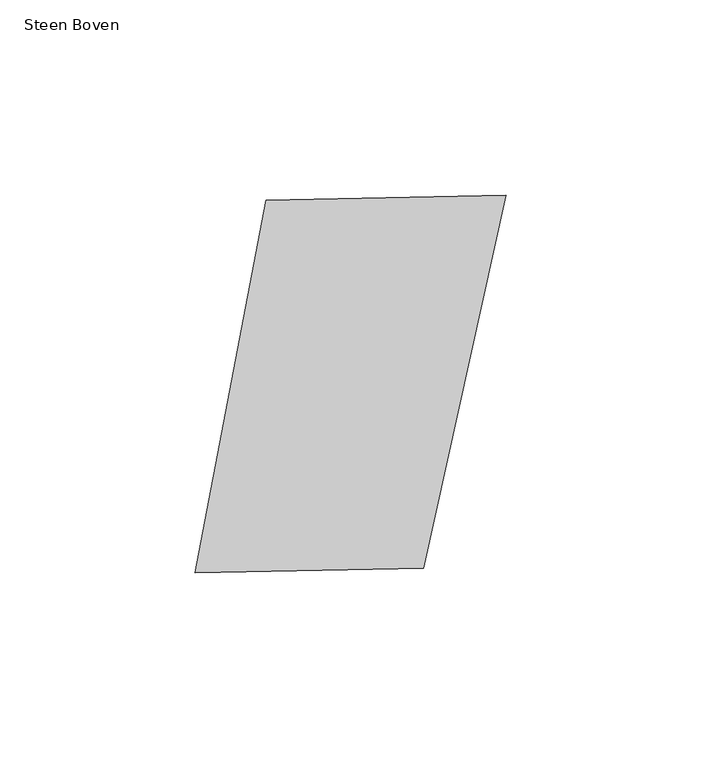
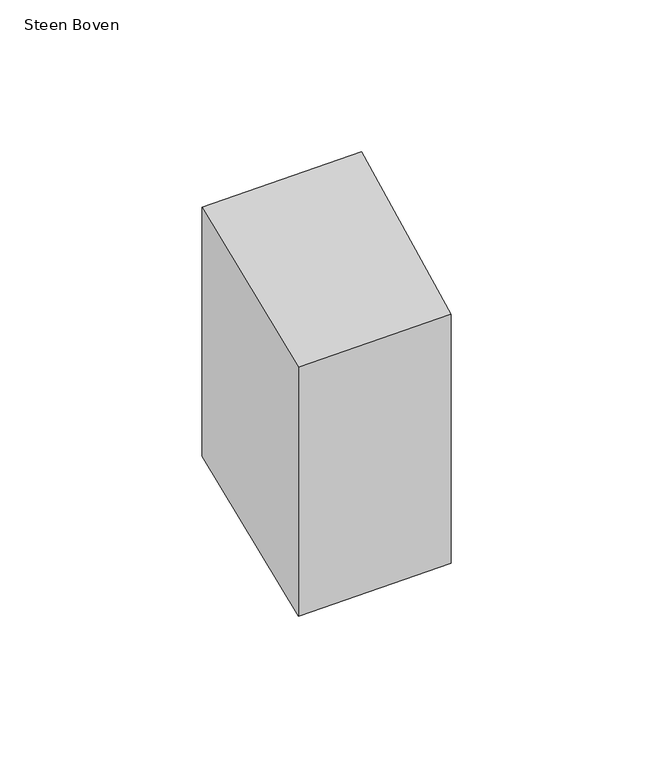
"""IFC4 building model written with IfcOpenShell, lengths in millimetres: proxy geometry, 00_GMA_steen_versie_4 : Steen Boven."""

import ifcopenshell
import ifcopenshell.guid

model = None  # the IFC model being written
_history = None  # IfcOwnerHistory: only IFC2X3 demands one
_inside = {}  # id of a spatial element -> (the spatial element, [elements in it])
_under = {}  # id of a project, library or spatial element -> (it, [spatial elements below it])
_declared = {}  # id of a project -> (the project, [libraries it declares])
_typed = {}  # id of a type object -> (the type object, [elements of that type])
_made_of = {}  # id of a material, layer set ... -> (it, [elements and type objects made of it])


def new_model(schema):
    """Start an empty IFC model of exactly this schema.

    Asked for "IFC4X3", IfcOpenShell would pick the latest addendum, in which some entities
    have other attributes; the version numbers below select the first issue.
    IFC2X3 requires an IfcOwnerHistory on every rooted entity: one is made here for all.
    """
    global model, _history
    if schema == "IFC4X3":
        model = ifcopenshell.file(schema_version=(4, 3, 0, 0))
    else:
        model = ifcopenshell.file(schema=schema)
    _inside.clear()
    _under.clear()
    _declared.clear()
    _typed.clear()
    _made_of.clear()
    _history = None
    if model.schema == "IFC2X3":
        org = make("IfcOrganization", Name="unknown")
        user = make(
            "IfcPersonAndOrganization",
            ThePerson=make("IfcPerson", FamilyName="unknown"),
            TheOrganization=org,
        )
        app = make(
            "IfcApplication",
            ApplicationDeveloper=org,
            Version="unknown",
            ApplicationFullName="unknown",
            ApplicationIdentifier="unknown",
        )
        _history = make(
            "IfcOwnerHistory",
            OwningUser=user,
            OwningApplication=app,
            ChangeAction="ADDED",
            CreationDate=0,
        )
    return model


def make(cls, **values):
    """One entity of the class cls with the attributes given. An attribute that is None is left unset."""
    return model.create_entity(
        cls, **{name: value for name, value in values.items() if value is not None}
    )


def rooted(cls, **values):
    """An entity with a GlobalId (a new one), such as an element, a storey or a relation."""
    return make(cls, GlobalId=ifcopenshell.guid.new(), OwnerHistory=_history, **values)


def si_unit(unit_type, name, prefix=None):
    """IfcSIUnit, for example si_unit("LENGTHUNIT", "METRE", prefix="MILLI")."""
    return make("IfcSIUnit", UnitType=unit_type, Prefix=prefix, Name=name)


def assignment(units):
    """IfcUnitAssignment: the units of a project."""
    return None if units is None else make("IfcUnitAssignment", Units=units)


def point(xyz):
    """IfcCartesianPoint."""
    return None if xyz is None else make("IfcCartesianPoint", Coordinates=xyz)


def direction(xyz):
    """IfcDirection."""
    return None if xyz is None else make("IfcDirection", DirectionRatios=xyz)


def frame(location, z_axis=None, x_axis=None):
    """IfcAxis2Placement3D, a coordinate frame: its origin and axes. An axis left out is left unset."""
    return make(
        "IfcAxis2Placement3D",
        Location=point(location),
        Axis=direction(z_axis),
        RefDirection=direction(x_axis),
    )


def origin():
    """The frame at (0, 0, 0) with its axes left unset."""
    return frame((0.0, 0.0, 0.0))


def origin_with_axes():
    """The frame at (0, 0, 0) with the z axis (0, 0, 1) and the x axis (1, 0, 0) written out."""
    return frame((0.0, 0.0, 0.0), z_axis=(0.0, 0.0, 1.0), x_axis=(1.0, 0.0, 0.0))


def place(relative_to, where):
    """IfcLocalPlacement: puts the frame where relative to a parent placement (None: the world)."""
    return make(
        "IfcLocalPlacement", PlacementRelTo=relative_to, RelativePlacement=where
    )


def context(
    kind, dimensions, precision=None, world=None, true_north=None, identifier=None
):
    """IfcGeometricRepresentationContext, for example the 3D "Model" context."""
    return make(
        "IfcGeometricRepresentationContext",
        ContextIdentifier=identifier,
        ContextType=kind,
        CoordinateSpaceDimension=dimensions,
        Precision=precision,
        WorldCoordinateSystem=world,
        TrueNorth=true_north,
    )


def project(units=None, contexts=None):
    """IfcProject with its units and contexts."""
    return rooted(
        "IfcProject",
        Name="project",
        RepresentationContexts=contexts,
        UnitsInContext=assignment(units),
    )


def spatial(cls, under=None, at=None, **own):
    """A site, building, storey or space (cls), placed at a placement, below another one or the project."""
    s = rooted(cls, ObjectPlacement=at, **own)
    if under is not None:
        _under.setdefault(under.id(), (under, []))[1].append(s)
    return s


def polyline(points):
    """IfcPolyline through the points."""
    return make("IfcPolyline", Points=[point(p) for p in points])


def outline(outer, holes=None, kind="AREA"):
    """IfcArbitraryClosedProfileDef: a profile drawn as a closed curve; with holes, ...WithVoids."""
    if holes is None:
        return make("IfcArbitraryClosedProfileDef", ProfileType=kind, OuterCurve=outer)
    return make(
        "IfcArbitraryProfileDefWithVoids",
        ProfileType=kind,
        OuterCurve=outer,
        InnerCurves=holes,
    )


def extrude(swept, where, along, depth):
    """IfcExtrudedAreaSolid: the profile swept, set in the frame where, extruded along a direction by depth."""
    return make(
        "IfcExtrudedAreaSolid",
        SweptArea=swept,
        Position=where,
        ExtrudedDirection=direction(along),
        Depth=depth,
    )


def shape(context_of_items, identifier, shape_type, items):
    """IfcShapeRepresentation: the items that make up one representation, for example the "Body"."""
    return make(
        "IfcShapeRepresentation",
        ContextOfItems=context_of_items,
        RepresentationIdentifier=identifier,
        RepresentationType=shape_type,
        Items=items,
    )


def source(mapping_origin, context_of_items, identifier, shape_type, items):
    """IfcRepresentationMap: a shape defined once, which mapped items show again and again."""
    return make(
        "IfcRepresentationMap",
        MappingOrigin=mapping_origin,
        MappedRepresentation=shape(context_of_items, identifier, shape_type, items),
    )


def transform(
    local_origin,
    x_axis=None,
    y_axis=None,
    z_axis=None,
    scale=None,
    scale2=None,
    scale3=None,
    uniform=True,
):
    """IfcCartesianTransformationOperator3D, or its non-uniform kind. x_axis, y_axis, z_axis: its Axis1, 2, 3."""
    if uniform:
        return make(
            "IfcCartesianTransformationOperator3D",
            Axis1=direction(x_axis),
            Axis2=direction(y_axis),
            LocalOrigin=point(local_origin),
            Scale=scale,
            Axis3=direction(z_axis),
        )
    return make(
        "IfcCartesianTransformationOperator3DnonUniform",
        Axis1=direction(x_axis),
        Axis2=direction(y_axis),
        LocalOrigin=point(local_origin),
        Scale=scale,
        Axis3=direction(z_axis),
        Scale2=scale2,
        Scale3=scale3,
    )


def mapped(mapping_source, mapping_target):
    """IfcMappedItem: shows the shape of a source again, moved by a transform."""
    return make(
        "IfcMappedItem", MappingSource=mapping_source, MappingTarget=mapping_target
    )


def made_of(thing, what):
    """Note that an element or type object is made of a material, layer set ...; save() writes the relation."""
    if what is not None:
        _made_of.setdefault(what.id(), (what, []))[1].append(thing)
    return thing


def element(
    cls,
    number,
    at=None,
    inside=None,
    cuts=None,
    type_object=None,
    material=None,
    context=None,
    identifier="Body",
    shape_type=None,
    held_by="IfcProductDefinitionShape",
    body=None,
    shapes=None,
    **own,
):
    """One element of the class cls, such as IfcWall. Its Tag is "e" and its number.

    at: its placement. inside: the storey or other place that contains it. cuts: it is an
    opening in that element (IfcRelVoidsElement). A single representation is given by context,
    identifier, shape_type and body (its items); several are given by shapes. held_by: the class
    of the entity that holds the representations. save() writes the other relations.
    """
    e = rooted(cls, Tag="e%d" % number, ObjectPlacement=at, **own)
    if body is not None:
        shapes = [shape(context, identifier, shape_type, body)]
    if shapes is not None:
        e.Representation = make(held_by, Representations=shapes)
    if inside is not None:
        _inside.setdefault(inside.id(), (inside, []))[1].append(e)
    if cuts is not None:
        rooted(
            "IfcRelVoidsElement", RelatingBuildingElement=cuts, RelatedOpeningElement=e
        )
    if type_object is not None:
        _typed.setdefault(type_object.id(), (type_object, []))[1].append(e)
    return made_of(e, material)


def aggregate(whole, parts):
    """IfcRelAggregates: a whole, such as a stair, and the parts it consists of."""
    return rooted("IfcRelAggregates", RelatingObject=whole, RelatedObjects=parts)


def save(model, path):
    """Write the relations noted so far, then the file.

    IfcRelAggregates (storeys below a building ...), IfcRelContainedInSpatialStructure (elements
    in a storey), IfcRelDefinesByType, IfcRelAssociatesMaterial and IfcRelDeclares: one each for
    every whole, place, type object, material and project.
    """
    for whole, parts in _under.values():
        aggregate(whole, parts)
    for where, things in _inside.values():
        rooted(
            "IfcRelContainedInSpatialStructure",
            RelatedElements=things,
            RelatingStructure=where,
        )
    for kind, things in _typed.values():
        rooted("IfcRelDefinesByType", RelatedObjects=things, RelatingType=kind)
    for what, things in _made_of.values():
        rooted("IfcRelAssociatesMaterial", RelatedObjects=things, RelatingMaterial=what)
    for by, libraries in _declared.values():
        rooted("IfcRelDeclares", RelatingContext=by, RelatedDefinitions=libraries)
    model.write(path)


def steen_boven_6947bcb0(model_context):
    return source(origin(), model_context, "Body", "SweptSolid", [
        extrude(outline(polyline([(111.6106463, 118.7393628), (90.5723202, 23.1219032), (31.8817785, 21.8754361), (50.196504, 117.4080049), (111.6106463, 118.7393628)])), origin_with_axes(), (0.0, 0.0, 1.0), 100.0),
    ])


if __name__ == "__main__":
    model = new_model("IFC4")
    model_context = context("Model", 3, world=origin())
    ifc_project = project(units=[si_unit("LENGTHUNIT", "METRE", prefix="MILLI")], contexts=[model_context])
    site = spatial("IfcSite", under=ifc_project)
    building = spatial("IfcBuilding", under=site)
    placement = place(None, origin())
    steen_boven_shape = steen_boven_6947bcb0(model_context)
    element("IfcBuildingElementProxy", 1, Name="00_GMA_steen_versie_4 : Steen Boven", ObjectType="00_GMA_steen_versie_4 : Steen Boven", at=placement, inside=building, context=model_context, shape_type="MappedRepresentation", body=[
        mapped(steen_boven_shape, transform((0.0, 0.0, 0.0), x_axis=(1.0, 0.0, 0.0), y_axis=(0.0, 1.0, 0.0), z_axis=(0.0, 0.0, 1.0))),
    ])
    save(model, "model.ifc")

# Revit data of these elements
# Type "00_GMA_steen_versie_4 : Steen Boven"
#   StootVoegHalfBoven [instance default] = 5 mm
#   StootVoegHalf [instance default] = 5 mm
#   StootVoegBreedteOnder = 10 mm
#   StootVoegBreedteBoven = 10 mm
#   Steendikte = 100 mm
#   LintVoegOnderHalf = 5 mm
#   LintVoegOnder = 10 mm
#   LintVoegBovenHalf = 0 mm
#   LintVoegBoven = 0 mm
#   materiaal = none
#   MateriaalVoeg = none
#   Default Elevation = 0
